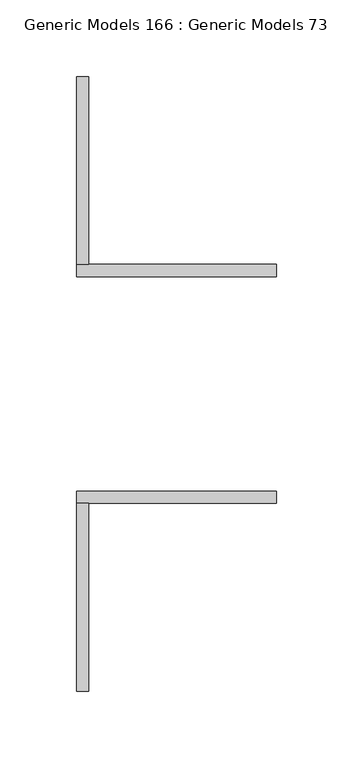
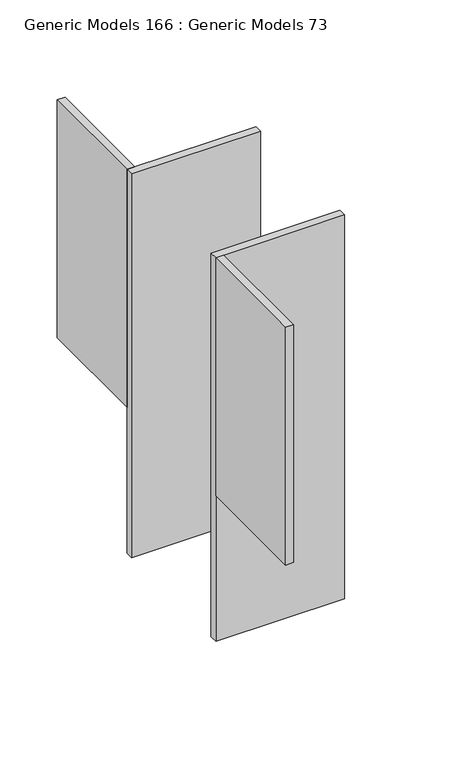
"""IFC4 building model written with IfcOpenShell, lengths in millimetres: proxy geometry, Generic Models 166 : Generic Models 73."""

from ifc_helpers import new_model, si_unit, frame, origin, place, context, project, spatial, polyline, outline, extrude, source, transform, mapped, element, save


def generic_models_166_generic_models_73_e4726cc4(model_context):
    return source(origin(), model_context, "Body", "SweptSolid", [
        extrude(outline(polyline([(31918.2596032, 30574.3156612), (31910.3221032, 30574.3156612), (31910.3221032, 30696.5531612), (31918.2596032, 30696.5531612), (31918.2596032, 30574.3156612)])), frame((0.0, 0.0, 271626.0125), z_axis=(0.0, 0.0, 1.0), x_axis=(1.0, 0.0, 0.0)), (0.0, 0.0, 1.0), 254.0),
        extrude(outline(polyline([(31910.3221032, 30974.3656612), (31918.2596032, 30974.3656612), (31918.2596032, 30852.1281612), (31910.3221032, 30852.1281612), (31910.3221032, 30974.3656612)])), frame((0.0, 0.0, 271626.0125), z_axis=(0.0, 0.0, 1.0), x_axis=(1.0, 0.0, 0.0)), (0.0, 0.0, 1.0), 254.0),
        extrude(outline(polyline([(32040.4971032, 30852.1281612), (32040.4971032, 30844.1906612), (31910.3221032, 30844.1906612), (31910.3221032, 30852.1281612), (32040.4971032, 30852.1281612)])), frame((0.0, 0.0, 271470.4375), z_axis=(0.0, 0.0, 1.0), x_axis=(1.0, 0.0, 0.0)), (0.0, 0.0, 1.0), 409.575),
        extrude(outline(polyline([(32040.4971032, 30704.4906612), (32040.4971032, 30696.5531612), (31910.3221032, 30696.5531612), (31910.3221032, 30704.4906612), (32040.4971032, 30704.4906612)])), frame((0.0, 0.0, 271470.4375), z_axis=(0.0, 0.0, 1.0), x_axis=(1.0, 0.0, 0.0)), (0.0, 0.0, 1.0), 409.575),
    ])


if __name__ == "__main__":
    model = new_model("IFC4")
    model_context = context("Model", 3, world=origin())
    ifc_project = project(units=[si_unit("LENGTHUNIT", "METRE", prefix="MILLI")], contexts=[model_context])
    site = spatial("IfcSite", under=ifc_project)
    building = spatial("IfcBuilding", under=site)
    placement = place(None, origin())
    generic_models_166_generic_models_73_shape = generic_models_166_generic_models_73_e4726cc4(model_context)
    element("IfcBuildingElementProxy", 1, Name="Generic Models 166 : Generic Models 73", ObjectType="Generic Models 166 : Generic Models 73", at=placement, inside=building, context=model_context, shape_type="MappedRepresentation", body=[
        mapped(generic_models_166_generic_models_73_shape, transform((0.0, 0.0, 0.0), x_axis=(1.0, 0.0, 0.0), y_axis=(0.0, 1.0, 0.0), z_axis=(0.0, 0.0, 1.0))),
    ])
    save(model, "model.ifc")

# Revit data of these elements
# Element 1 (IfcBuildingElementProxy, "Generic Models 166 : Generic Models 73")
#   Materials on its faces: "5 1/8 x 10 x 0 5/16\" PLATE W/ 3 1\"DIA. THRU BOLTS", "5/16 x 9 x 0'-11\" SIDE PLATES  CAP\nW/ 2 3/4\"DIA. THRU BOLTS"
# Materials
#   "5 1/8 x 10 x 0 5/16\" PLATE W/ 3 1\"DIA. THRU BOLTS": class "Metal", colour RGB 199 199 199, transparency 0, Description = "Carbon steel", Cost = 0
#   "5/16 x 9 x 0'-11\" SIDE PLATES  CAP\nW/ 2 3/4\"DIA. THRU BOLTS": class "Metal", colour RGB 199 199 199, transparency 0, Description = "Carbon steel", Cost = 0
